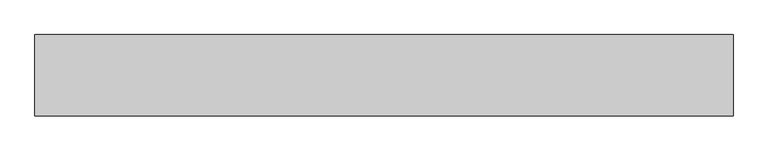
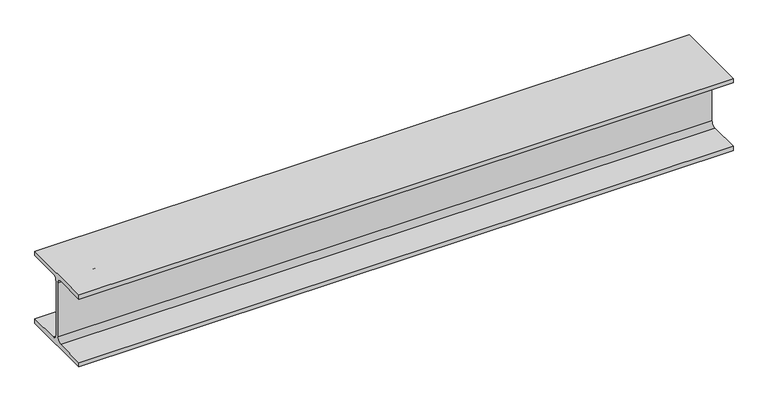
"""IFC4 building model written with IfcOpenShell, lengths in millimetres: beam geometry, 0912_Steel Framing_H-KSD3502 : H_SB_ASB_H-200x200x8x12."""

from ifc_helpers import new_model, si_unit, point, frame, frame_2d, origin, place, context, project, spatial, polyline, circle_curve, trimmed, segment, composite_curve, outline, extrude, source, transform, mapped, element, save


def beam_db06266e(model_context):
    return source(origin(), model_context, "Body", "SweptSolid", [
        extrude(outline(composite_curve([segment(polyline([(100.0, -88.0), (100.0, -100.0), (-100.0, -100.0), (-100.0, -88.0), (-17.0, -88.0)]), True, "CONTINUOUS"), segment(trimmed(circle_curve(frame_2d((-17.0, -75.0)), 13.0), [point((-17.0, -88.0))], [point((-4.0, -75.0))], True, "CARTESIAN"), True, "CONTINUOUS"), segment(polyline([(-4.0, -75.0), (-4.0, 75.0)]), True, "CONTINUOUS"), segment(trimmed(circle_curve(frame_2d((-17.0, 75.0)), 13.0), [point((-4.0, 75.0))], [point((-17.0, 88.0))], True, "CARTESIAN"), True, "CONTINUOUS"), segment(polyline([(-17.0, 88.0), (-100.0, 88.0), (-100.0, 100.0), (100.0, 100.0), (100.0, 88.0), (17.0, 88.0)]), True, "CONTINUOUS"), segment(trimmed(circle_curve(frame_2d((17.0, 75.0)), 13.0), [point((17.0, 88.0))], [point((4.0, 75.0))], True, "CARTESIAN"), True, "CONTINUOUS"), segment(polyline([(4.0, 75.0), (4.0, -75.0)]), True, "CONTINUOUS"), segment(trimmed(circle_curve(frame_2d((17.0, -75.0)), 13.0), [point((4.0, -75.0))], [point((17.0, -88.0))], True, "CARTESIAN"), True, "CONTINUOUS"), segment(polyline([(17.0, -88.0), (100.0, -88.0)]), True, "CONTINUOUS")], self_intersect=False)), frame((-974.6172257, 0.0, 0.0), z_axis=(1.0, 0.0, 0.0), x_axis=(0.0, 1.0, 0.0)), (0.0, 0.0, 1.0), 1716.9069192),
    ])


if __name__ == "__main__":
    model = new_model("IFC4")
    model_context = context("Model", 3, world=origin())
    ifc_project = project(units=[si_unit("LENGTHUNIT", "METRE", prefix="MILLI")], contexts=[model_context])
    site = spatial("IfcSite", under=ifc_project)
    building = spatial("IfcBuilding", under=site)
    placement = place(None, origin())
    beam_shape = beam_db06266e(model_context)
    element("IfcBeam", 1, ObjectType="0912_Steel Framing_H-KSD3502 : H_SB_ASB_H-200x200x8x12", at=placement, inside=building, context=model_context, shape_type="MappedRepresentation", body=[
        mapped(beam_shape, transform((0.0, 0.0, 0.0), x_axis=(1.0, 0.0, 0.0), y_axis=(0.0, 1.0, 0.0), z_axis=(0.0, 0.0, 1.0))),
    ])
    save(model, "model.ifc")

# Revit data of these elements
# Type "0912_Steel Framing_H-KSD3502 : H_SB_ASB_H-200x200x8x12"
#   H_WM Code_1 = "S01AA002-00001 | Main Steel Structure Fabrication Work | Shelter/Building | Medium Steel - Standard (90KG/M>Weight≥30KG/M) | Material: (   )"
#   H_WM Code_2 = "S03AA028-00001 | Main Steel Structure Erection Work | Shelter/Building | Medium Steel (90KG/M>Weight≥30KG/M) | Material: (   )"
#   H_WM Code_3 = "S01AA010-00001 | Main Steel Structure Fabrication Work | Shelter/Building | Steel Painting/Coating | for Non-Fireproofed Steel Surface, Surface Preparation, Primer, Second & Final Coat | Material: (   )"
#   H_Q'ty Cal Type Tag = "SB-Q2"
#   Width = 20.0 cm
#   Web Thickness = 0.8 cm
#   Web Fillet = 1.3 cm
#   Warping Constant = 141000.0 cm⁶
#   W = 0
#   Torsional Moment of Inertia = 26.2485 cm⁴
#   Section Area = 63.53 cm²
#   Plastic Modulus weak axis = 244.0 cm³
#   Plastic Modulus strong axis = 525.0 cm³
#   Perimeter = 1.16 m²/m
#   Nominal Weight = 49.90 kgf/m
#   Moment of Inertia weak axis = 1600.00 cm⁴
#   Moment of Inertia strong axis = 4720.00 cm⁴
#   Height = 20.0 cm
#   Flange Thickness = 1.2 cm
#   Elastic Modulus weak axis = 160.0 cm³
#   Elastic Modulus strong axis = 472.0 cm³
#   Centroid Vertical = 10.0 cm
#   Centroid Horizontal = 10.0 cm
#   Ix = 47200000
#   Length [instance default] = 1.5240 m
#   Zx = 525000
#   b = 0.2000 m
#   h = 0.2000 m
#   r = 0.0130 m
#   s = 0.0080 m
#   t = 0.0120 m
#   A = 0.006353 m²
#   Structural Material [instance default] = Steel, 45-345
#   Assembly Code = ""
# Element 1 (IfcBeam, "0912_Steel Framing_H-KSD3502 : H_SB_ASB_H-200x200x8x12")
#   Structural Material = none
# Materials
#   "Steel, 45-345": class "Metal", colour RGB 189 187 185, transparency 0, Description = "Steel 345 MPa", Cost = 0
